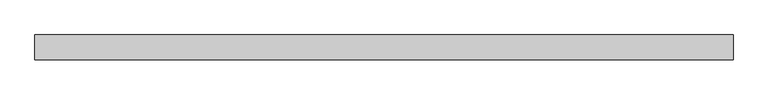
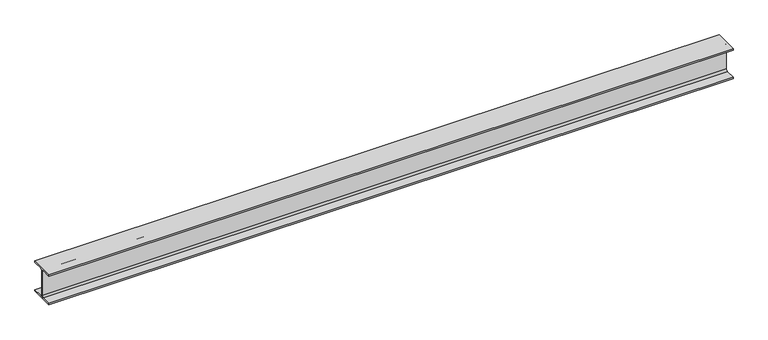
"""IFC4 building model written with IfcOpenShell, lengths in millimetres: beam geometry, 0912_Steel Framing_H-KSD3502 : H_SB_ASB_H-390x300x10x16."""

from ifc_helpers import new_model, si_unit, point, frame, frame_2d, origin, place, context, project, spatial, polyline, circle_curve, trimmed, segment, composite_curve, outline, extrude, source, transform, mapped, element, save


def beam_bbc4af74(model_context):
    return source(origin(), model_context, "Body", "SweptSolid", [
        extrude(outline(composite_curve([segment(polyline([(150.0, -179.0), (150.0, -195.0), (-150.0, -195.0), (-150.0, -179.0), (-27.0, -179.0)]), True, "CONTINUOUS"), segment(trimmed(circle_curve(frame_2d((-27.0, -157.0)), 22.0), [point((-27.0, -179.0))], [point((-5.0, -157.0))], True, "CARTESIAN"), True, "CONTINUOUS"), segment(polyline([(-5.0, -157.0), (-5.0, 157.0)]), True, "CONTINUOUS"), segment(trimmed(circle_curve(frame_2d((-27.0, 157.0)), 22.0), [point((-5.0, 157.0))], [point((-27.0, 179.0))], True, "CARTESIAN"), True, "CONTINUOUS"), segment(polyline([(-27.0, 179.0), (-150.0, 179.0), (-150.0, 195.0), (150.0, 195.0), (150.0, 179.0), (27.0, 179.0)]), True, "CONTINUOUS"), segment(trimmed(circle_curve(frame_2d((27.0, 157.0)), 22.0), [point((27.0, 179.0))], [point((5.0, 157.0))], True, "CARTESIAN"), True, "CONTINUOUS"), segment(polyline([(5.0, 157.0), (5.0, -157.0)]), True, "CONTINUOUS"), segment(trimmed(circle_curve(frame_2d((27.0, -157.0)), 22.0), [point((5.0, -157.0))], [point((27.0, -179.0))], True, "CARTESIAN"), True, "CONTINUOUS"), segment(polyline([(27.0, -179.0), (150.0, -179.0)]), True, "CONTINUOUS")], self_intersect=False)), frame((-4237.2999994, 0.0, 0.0), z_axis=(1.0, 0.0, 0.0), x_axis=(0.0, 1.0, 0.0)), (0.0, 0.0, 1.0), 8474.5999988),
    ])


if __name__ == "__main__":
    model = new_model("IFC4")
    model_context = context("Model", 3, world=origin())
    ifc_project = project(units=[si_unit("LENGTHUNIT", "METRE", prefix="MILLI")], contexts=[model_context])
    site = spatial("IfcSite", under=ifc_project)
    building = spatial("IfcBuilding", under=site)
    placement = place(None, origin())
    beam_shape = beam_bbc4af74(model_context)
    element("IfcBeam", 1, ObjectType="0912_Steel Framing_H-KSD3502 : H_SB_ASB_H-390x300x10x16", at=placement, inside=building, context=model_context, shape_type="MappedRepresentation", body=[
        mapped(beam_shape, transform((0.0, 0.0, 0.0), x_axis=(1.0, 0.0, 0.0), y_axis=(0.0, 1.0, 0.0), z_axis=(0.0, 0.0, 1.0))),
    ])
    save(model, "model.ifc")

# Revit data of these elements
# Type "0912_Steel Framing_H-KSD3502 : H_SB_ASB_H-390x300x10x16"
#   H_WM Code_1 = "S01AA001-00001 | Main Steel Structure Fabrication Work | Shelter/Building | Heavy Steel - Standard (Weight≥90KG/M) | Material: (   )"
#   H_WM Code_2 = "S03AA027-00001 | Main Steel Structure Erection Work | Shelter/Building | Heavy Steel (Weight≥90KG/M) | Material: (   )"
#   H_WM Code_3 = "S01AA010-00001 | Main Steel Structure Fabrication Work | Shelter/Building | Steel Painting/Coating | for Non-Fireproofed Steel Surface, Surface Preparation, Primer, Second & Final Coat | Material: (   )"
#   H_Q'ty Cal Type Tag = "SB-Q2"
#   Width = 30.0 cm
#   Web Thickness = 1.0 cm
#   Web Fillet = 2.2 cm
#   Warping Constant = 2520000.0 cm⁶
#   W = 0
#   Torsional Moment of Inertia = 94.3867 cm⁴
#   Section Area = 136.0 cm²
#   Plastic Modulus weak axis = 733.0 cm³
#   Plastic Modulus strong axis = 2190.0 cm³
#   Perimeter = 1.92 m²/m
#   Nominal Weight = 107.00 kgf/m
#   Moment of Inertia weak axis = 7210.00 cm⁴
#   Moment of Inertia strong axis = 38700.00 cm⁴
#   Height = 39.0 cm
#   Flange Thickness = 1.6 cm
#   Elastic Modulus weak axis = 481.0 cm³
#   Elastic Modulus strong axis = 1980.0 cm³
#   Centroid Vertical = 19.5 cm
#   Centroid Horizontal = 15.0 cm
#   Ix = 387000000
#   Length [instance default] = 1.5240 m
#   Zx = 2190000
#   b = 0.3000 m
#   h = 0.3900 m
#   r = 0.0220 m
#   s = 0.0100 m
#   t = 0.0160 m
#   A = 0.0136 m²
#   Structural Material [instance default] = Steel, 45-345
#   Assembly Code = ""
# Element 1 (IfcBeam, "0912_Steel Framing_H-KSD3502 : H_SB_ASB_H-390x300x10x16")
#   Structural Material = none
# Materials
#   "Steel, 45-345": class "Metal", colour RGB 189 187 185, transparency 0, Description = "Steel 345 MPa", Cost = 0
